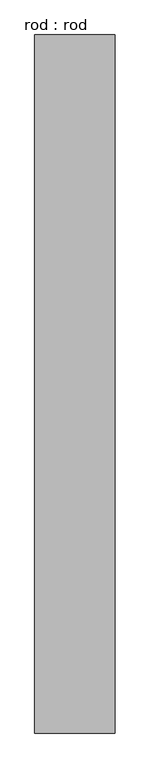
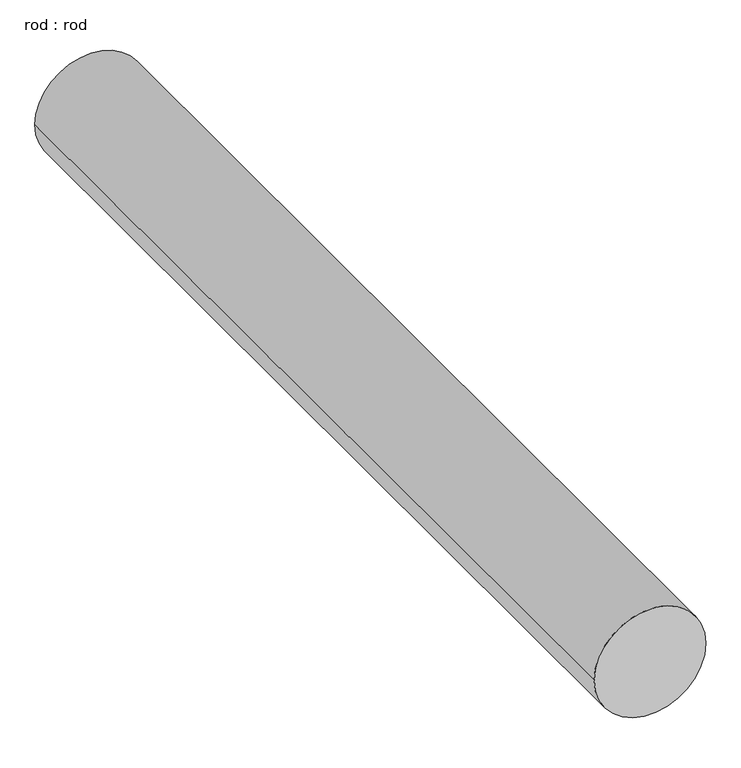
"""IFC4 building model written with IfcOpenShell, lengths in millimetres: proxy geometry, rod : rod."""

from ifc_helpers import new_model, si_unit, point, frame, frame_2d, origin, place, context, project, spatial, circle_curve, trimmed, segment, composite_curve, outline, extrude, source, transform, mapped, element, save


def rod_rod_1fbcbc39(model_context):
    return source(origin(), model_context, "Body", "SweptSolid", [
        extrude(outline(composite_curve([segment(trimmed(circle_curve(frame_2d((0.0108462, 0.0)), 200.0), [point((0.0108462, 200.0))], [point((0.0108462, -200.0))], False, "CARTESIAN"), True, "CONTINUOUS"), segment(trimmed(circle_curve(frame_2d((0.0108462, 0.0)), 200.0), [point((0.0108462, -200.0))], [point((0.0108462, 200.0))], False, "CARTESIAN"), True, "CONTINUOUS")], self_intersect=False)), frame((0.0, 2357.0143296, 0.0), z_axis=(0.0, 1.0, 0.0), x_axis=(0.0, 0.0, 1.0)), (0.0, 0.0, 1.0), 3471.4285714),
    ])


if __name__ == "__main__":
    model = new_model("IFC4")
    model_context = context("Model", 3, world=origin())
    ifc_project = project(units=[si_unit("LENGTHUNIT", "METRE", prefix="MILLI")], contexts=[model_context])
    site = spatial("IfcSite", under=ifc_project)
    building = spatial("IfcBuilding", under=site)
    placement = place(None, origin())
    rod_rod_shape = rod_rod_1fbcbc39(model_context)
    element("IfcBuildingElementProxy", 1, Name="rod : rod", ObjectType="rod : rod", at=placement, inside=building, context=model_context, shape_type="MappedRepresentation", body=[
        mapped(rod_rod_shape, transform((0.0, 0.0, 0.0), x_axis=(1.0, 0.0, 0.0), y_axis=(0.0, 1.0, 0.0), z_axis=(0.0, 0.0, 1.0))),
    ])
    save(model, "model.ifc")

# Revit data of these elements
# Type "rod : rod"
#   Default Elevation = 0
